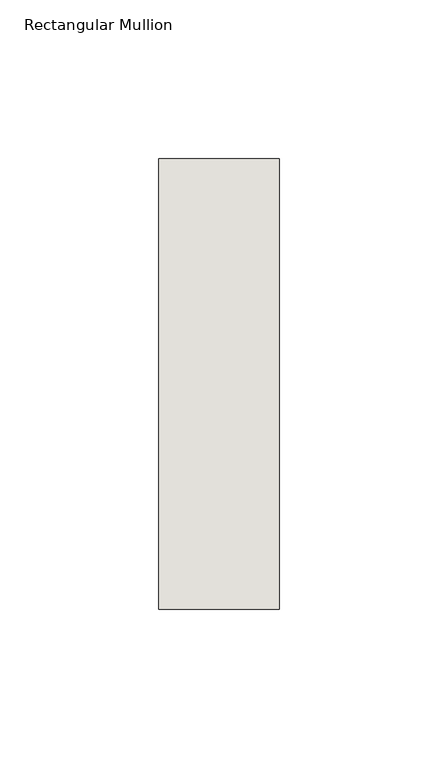
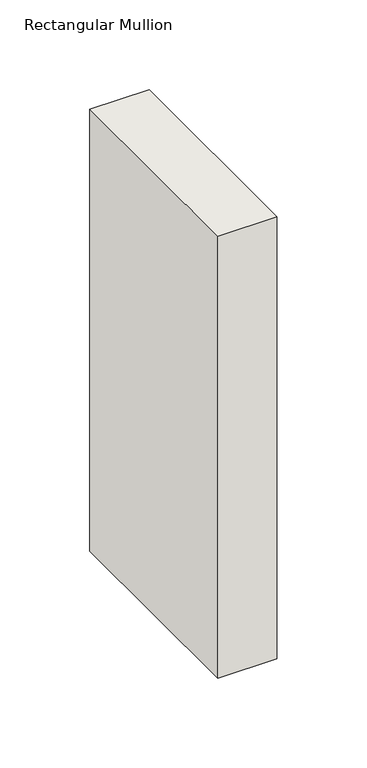
"""IFC4 building model written with IfcOpenShell, lengths in millimetres: wall geometry, Rectangular Mullion : NLRS_21_CWM_hsb-regel 38x142_gen_rsf."""

from ifc_helpers import new_model, si_unit, frame, origin, place, context, project, spatial, polyline, outline, extrude, source, transform, mapped, element, save


def rectangular_mullion_25b390b2(model_context):
    return source(origin(), model_context, "Body", "SweptSolid", [
        extrude(outline(polyline([(-38.0, -71.0), (-38.0, 71.0), (0.0, 71.0), (0.0, -71.0), (-38.0, -71.0)])), frame((0.0, 0.0, -300.0), z_axis=(0.0, 0.0, 1.0), x_axis=(1.0, 0.0, 0.0)), (0.0, 0.0, 1.0), 300.0),
    ])


if __name__ == "__main__":
    model = new_model("IFC4")
    model_context = context("Model", 3, world=origin())
    ifc_project = project(units=[si_unit("LENGTHUNIT", "METRE", prefix="MILLI")], contexts=[model_context])
    site = spatial("IfcSite", under=ifc_project)
    building = spatial("IfcBuilding", under=site)
    placement = place(None, origin())
    rectangular_mullion_shape = rectangular_mullion_25b390b2(model_context)
    element("IfcWall", 1, ObjectType="Rectangular Mullion : NLRS_21_CWM_hsb-regel 38x142_gen_rsf", at=placement, inside=building, context=model_context, shape_type="MappedRepresentation", body=[
        mapped(rectangular_mullion_shape, transform((0.0, 0.0, 0.0), x_axis=(1.0, 0.0, 0.0), y_axis=(0.0, 1.0, 0.0), z_axis=(0.0, 0.0, 1.0))),
    ])
    save(model, "model.ifc")

# Revit data of these elements
# Type "Rectangular Mullion : NLRS_21_CWM_hsb-regel 38x142_gen_rsf"
#   Type IfcGUID = "07M7mRoiH1CR8m_RSKIwpF"
#   Assembly Code = "21.10"
#   IfcExportAs = "IfcWall"
#   built-in parameter 1007322 = 0.465879 (stored number, unit not read)
#   built-in parameter 1007321 = 0.062336 (stored number, unit not read)
#   built-in parameter 1007320 = 0.062336 (stored number, unit not read)
# Element 1 (IfcWall, "Rectangular Mullion : NLRS_21_CWM_hsb-regel 38x142_gen_rsf")
#   Materials on its faces: "NLRS_i2_hout naaldhout vuren_gen_rsf"
# Materials
#   "NLRS_i2_hout naaldhout vuren_gen_rsf": class "I - Hout", colour RGB 234 199 147, transparency 0, Keynote = "i2", Manufacturer = "Revit Standards Foundation", URL = "www.revitstandards.org", Description = "hout vuren", Cost = 0
